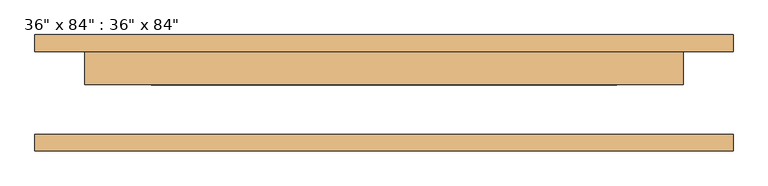
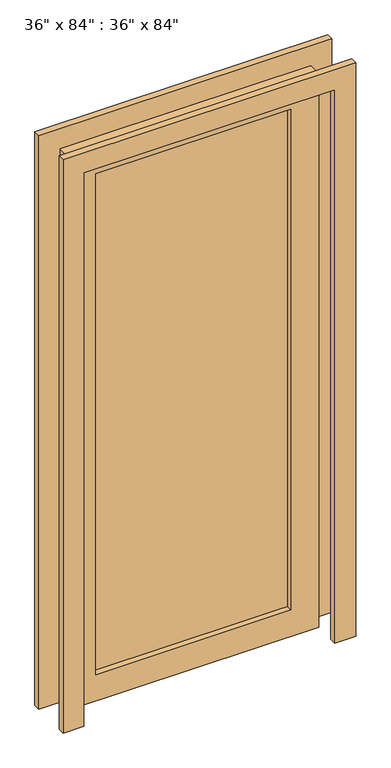
"""IFC4 building model written with IfcOpenShell, lengths in millimetres: door geometry."""

from ifc_helpers import new_model, si_unit, frame, origin, place, context, project, spatial, polyline, outline, extrude, source, transform, mapped, element, save


def door_fc661d27(model_context):
    return source(origin(), model_context, "Body", "SweptSolid", [
        extrude(outline(polyline([(0.0, -457.2), (2133.6, -457.2), (2133.6, 457.2), (0.0, 457.2), (0.0, 533.4), (2209.8, 533.4), (2209.8, -533.4), (0.0, -533.4), (0.0, -457.2)])), frame((0.0, -88.9, 0.0), z_axis=(0.0, 1.0, 0.0), x_axis=(0.0, 0.0, 1.0)), (0.0, 0.0, 1.0), 25.4),
        extrude(outline(polyline([(0.0, -457.2), (2133.6, -457.2), (2133.6, 457.2), (0.0, 457.2), (0.0, 533.4), (2209.8, 533.4), (2209.8, -533.4), (0.0, -533.4), (0.0, -457.2)])), frame((0.0, 63.5, 0.0), z_axis=(0.0, 1.0, 0.0), x_axis=(0.0, 0.0, 1.0)), (0.0, 0.0, 1.0), 25.4),
        extrude(outline(polyline([(-355.6, 41.275), (355.6, 41.275), (355.6, 34.925), (-355.6, 34.925), (-355.6, 41.275)])), frame((0.0, 0.0, 101.6), z_axis=(0.0, 0.0, 1.0), x_axis=(1.0, 0.0, 0.0)), (0.0, 0.0, 1.0), 1930.4),
        extrude(outline(polyline([(0.0, -457.2), (0.0, 457.2), (2133.6, 457.2), (2133.6, -457.2), (0.0, -457.2)]), holes=[polyline([(101.6, 355.6), (101.6, -355.6), (2032.0, -355.6), (2032.0, 355.6), (101.6, 355.6)])]), frame((0.0, 12.7, 0.0), z_axis=(0.0, 1.0, 0.0), x_axis=(0.0, 0.0, 1.0)), (0.0, 0.0, 1.0), 50.8),
    ])


if __name__ == "__main__":
    model = new_model("IFC4")
    model_context = context("Model", 3, world=origin())
    ifc_project = project(units=[si_unit("LENGTHUNIT", "METRE", prefix="MILLI")], contexts=[model_context])
    site = spatial("IfcSite", under=ifc_project)
    building = spatial("IfcBuilding", under=site)
    placement = place(None, origin())
    door_shape = door_fc661d27(model_context)
    element("IfcDoor", 1, ObjectType="36\" x 84\" : 36\" x 84\"", at=placement, inside=building, context=model_context, shape_type="MappedRepresentation", body=[
        mapped(door_shape, transform((0.0, 0.0, 0.0), x_axis=(1.0, 0.0, 0.0), y_axis=(0.0, 1.0, 0.0), z_axis=(0.0, 0.0, 1.0))),
    ])
    save(model, "model.ifc")

# Revit data of these elements
# Type "36\" x 84\" : 36\" x 84\""
#   Type IfcGUID = "0MuvbwA9n44vt4gtWSRz3C"
#   Type Mark = "10"
#   Operation = "SINGLE_SWING_RIGHT"
#   NameOverride = "36\" x 84\":36\" x 84\":302032"
#   ObjectTypeOverride = "36\" x 84\""
#   Tag = "302032"
#   Reference = "36\" x 84\""
#   ThermalTransmittance = 3.7021 (stored number, unit not read)
#   IsExternal = no
